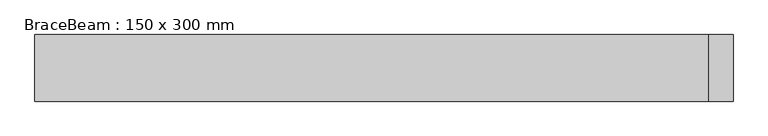
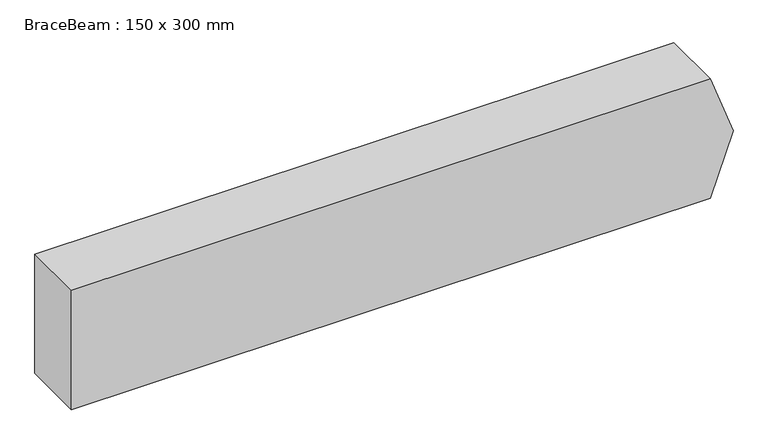
"""IFC4 building model written with IfcOpenShell, lengths in millimetres: beam geometry, BraceBeam : 150 x 300 mm."""

from ifc_helpers import new_model, si_unit, frame, origin, place, context, project, spatial, polyline, outline, extrude, source, transform, mapped, element, save


def bracebeam_150_x_300_mm_1b5e1667(model_context):
    return source(origin(), model_context, "Body", "SweptSolid", [
        extrude(outline(polyline([(150.0, -865.8540869), (-150.0, -865.8540869), (-150.0, 651.6318859), (0.0, 706.2274211), (150.0, 651.6318859), (150.0, -865.8540869)])), frame((0.0, -75.0, 0.0), z_axis=(0.0, 1.0, 0.0), x_axis=(0.0, 0.0, 1.0)), (0.0, 0.0, 1.0), 150.0),
    ])


if __name__ == "__main__":
    model = new_model("IFC4")
    model_context = context("Model", 3, world=origin())
    ifc_project = project(units=[si_unit("LENGTHUNIT", "METRE", prefix="MILLI")], contexts=[model_context])
    site = spatial("IfcSite", under=ifc_project)
    building = spatial("IfcBuilding", under=site)
    placement = place(None, origin())
    bracebeam_150_x_300_mm_shape = bracebeam_150_x_300_mm_1b5e1667(model_context)
    element("IfcBeam", 1, ObjectType="BraceBeam : 150 x 300 mm", at=placement, inside=building, context=model_context, shape_type="MappedRepresentation", body=[
        mapped(bracebeam_150_x_300_mm_shape, transform((0.0, 0.0, 0.0), x_axis=(1.0, 0.0, 0.0), y_axis=(0.0, 1.0, 0.0), z_axis=(0.0, 0.0, 1.0))),
    ])
    save(model, "model.ifc")

# Revit data of these elements
# Type "BraceBeam : 150 x 300 mm"
#   ExpertTruss = "Height\th\r\nWidth\tb"
#   Name [instance default] = ""
#   m [instance default] = 0 mm
#   ip_c_cut_control [instance default] = 1300 mm
#   ip_c_cut [instance default] = 1300 mm
#   h_fix [instance default] = 900 mm
#   d/2 [instance default] = 1750 mm
#   c_cut_incl [instance default] = -1000 mm
#   c_cut [instance default] = 0 mm
#   beta0_2 [instance default] = 90.00°
#   beta0_1 [instance default] = 90.00°
#   alfaMax [instance default] = 0.00°
#   alfa0_2 [instance default] = 90.00°
#   ZOffsetStr_0 [instance default] = 150 mm
#   ZOffsetStr [instance default] = 0 mm
#   ZOffsetEnd_0 [instance default] = 150 mm
#   ZOffsetEnd [instance default] = 0 mm
#   Beta2 [instance default] = 0.00°
#   Beta1 [instance default] = 0.00°
#   Alfa_str [instance default] = 0.00°
#   Alfa_cut_control [instance default] = 90.00°
#   Alfa_cut [instance default] = 90.00°
#   AlfaMAX [instance default] = 0.00°
#   Alfa2_0 [instance default] = 0.00°
#   Alfa2 [instance default] = 0.00°
#   Alfa1_0 [instance default] = 0.00°
#   Alfa1 [instance default] = 0.00°
#   A_max_Str [instance default] = 0.00°
#   h_void [instance default] = 3000 mm
#   beam_L_0 [instance default] = 100 mm
#   beam_L [instance default] = 0 mm
#   b_void [instance default] = 160 mm
#   alfa0_1 [instance default] = 90.00°
#   b = 150 mm
#   YOffsetStr [instance default] = 0 mm
#   YOffsetEnd [instance default] = 0 mm
#   XOffsetStr_0 [instance default] = 3500 mm
#   XOffsetStr [instance default] = 0 mm
#   XOffsetEnd_0 [instance default] = 3500 mm
#   XOffsetEnd [instance default] = 0 mm
#   L_void_0 [instance default] = 100 mm
#   L_void [instance default] = 0 mm
#   E2 [instance default] = 0.00°
#   E1 [instance default] = 0.00°
#   Length [instance default] = 3500 mm
#   h = 300 mm
#   Alfa [instance default] = 0.00°
#   A_max_End [instance default] = 0.00°
#   A_max [instance default] = 0.00°
#   A4 [instance default] = 0.00°
#   A3 [instance default] = 0.00°
#   A2 [instance default] = 0.00°
#   A1 [instance default] = 0.00°
#   BetaAngles [instance default] = no
#   Material [instance default] = Wood Standard
# Element 1 (IfcBeam, "BraceBeam : 150 x 300 mm")
#   d/2 = 865.854 mm
#   beta0_2 = 70.00°
#   alfaMax = 20.00°
#   alfa0_2 = 110.00°
#   Beta2 = -20.00°
#   AlfaMAX = 20.00°
#   Alfa2_0 = 20.00°
#   Alfa2 = 20.00°
#   h_void = 4091.911 mm
#   beam_L_0 = 873.529 mm
#   beam_L = 873.529 mm
#   XOffsetStr_0 = 1731.708 mm
#   XOffsetEnd_0 = 1572.082 mm
#   XOffsetEnd = 159.627 mm
#   L_void_0 = 2064.996 mm
#   L_void = 2064.996 mm
#   BetaAngles = yes
#   Materials on its faces: "Wood Standard"
# Materials
#   "Wood Standard": class "Drewno", colour RGB 196 146 67, transparency 0, Cost = 0
